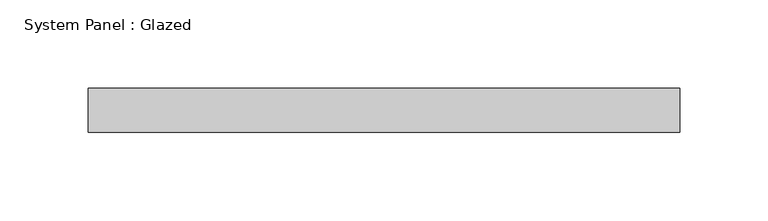
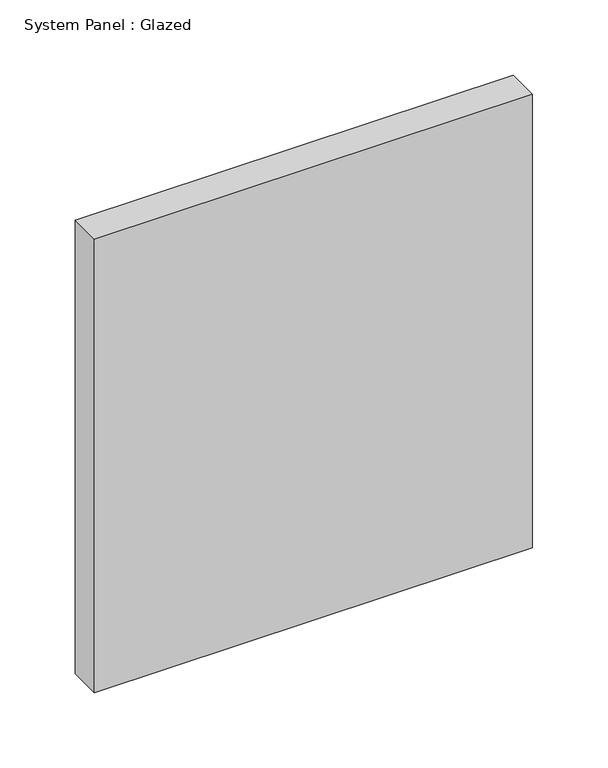
"""IFC4 building model written with IfcOpenShell, lengths in millimetres: plate geometry, System Panel : Glazed."""

from ifc_helpers import new_model, si_unit, origin, origin_with_axes, place, context, project, spatial, polyline, outline, extrude, source, transform, mapped, element, save


def system_panel_glazed_db55e23d(model_context):
    return source(origin(), model_context, "Body", "SweptSolid", [
        extrude(outline(polyline([(167.4242424, 24.5), (-167.4242424, 24.5), (-167.4242424, 49.5), (167.4242424, 49.5), (167.4242424, 24.5)])), origin_with_axes(), (0.0, 0.0, 1.0), 366.6666667),
    ])


if __name__ == "__main__":
    model = new_model("IFC4")
    model_context = context("Model", 3, world=origin())
    ifc_project = project(units=[si_unit("LENGTHUNIT", "METRE", prefix="MILLI")], contexts=[model_context])
    site = spatial("IfcSite", under=ifc_project)
    building = spatial("IfcBuilding", under=site)
    placement = place(None, origin())
    system_panel_glazed_shape = system_panel_glazed_db55e23d(model_context)
    element("IfcPlate", 1, ObjectType="System Panel : Glazed", at=placement, inside=building, context=model_context, shape_type="MappedRepresentation", body=[
        mapped(system_panel_glazed_shape, transform((0.0, 0.0, 0.0), x_axis=(1.0, 0.0, 0.0), y_axis=(0.0, 1.0, 0.0), z_axis=(0.0, 0.0, 1.0))),
    ])
    save(model, "model.ifc")

# Revit data of these elements
# Element 1 (IfcPlate, "System Panel : Glazed")
#   Materials on its faces: "Glass"
# Materials
#   "Glass": class "Glass", colour RGB 218 227 224, transparency 0.85, Description = "Soda Lime Glass", Cost = 0
